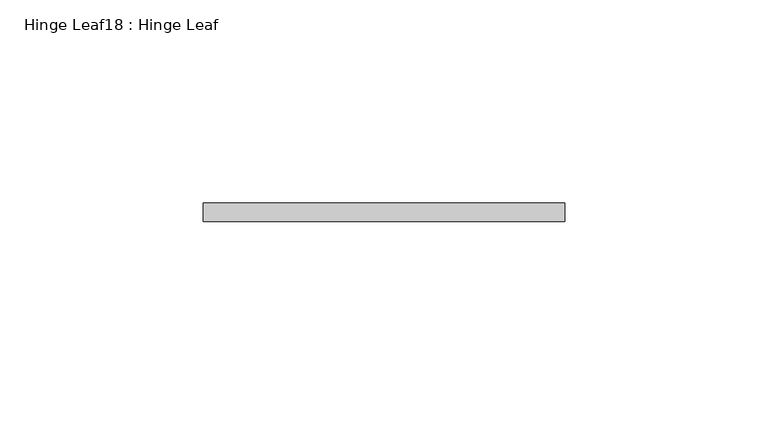
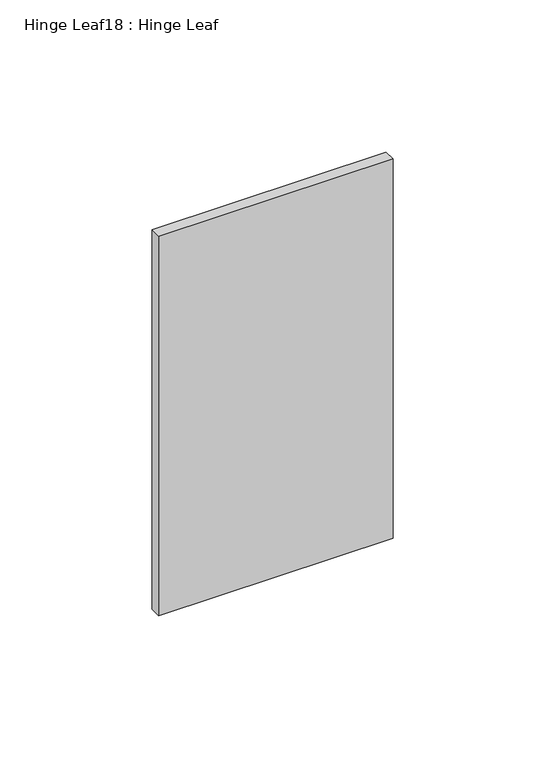
"""IFC4 building model written with IfcOpenShell, lengths in millimetres: proxy geometry, Hinge Leaf18 : Hinge Leaf."""

from ifc_helpers import new_model, si_unit, frame, origin, place, context, project, spatial, polyline, outline, extrude, source, transform, mapped, element, save


def hinge_leaf18_hinge_leaf_9b6187f5(model_context):
    return source(origin(), model_context, "Body", "SweptSolid", [
        extrude(outline(polyline([(587327.7934739, -534104.7943841), (587416.6934739, -534104.7943841), (587416.6934739, -534109.3663841), (587327.7934739, -534109.3663841), (587327.7934739, -534104.7943841)])), frame((0.0, 0.0, 1123.95), z_axis=(0.0, 0.0, 1.0), x_axis=(1.0, 0.0, 0.0)), (0.0, 0.0, 1.0), 152.4),
    ])


if __name__ == "__main__":
    model = new_model("IFC4")
    model_context = context("Model", 3, world=origin())
    ifc_project = project(units=[si_unit("LENGTHUNIT", "METRE", prefix="MILLI")], contexts=[model_context])
    site = spatial("IfcSite", under=ifc_project)
    building = spatial("IfcBuilding", under=site)
    placement = place(None, origin())
    hinge_leaf18_hinge_leaf_shape = hinge_leaf18_hinge_leaf_9b6187f5(model_context)
    element("IfcBuildingElementProxy", 1, Name="Hinge Leaf18 : Hinge Leaf", ObjectType="Hinge Leaf18 : Hinge Leaf", at=placement, inside=building, context=model_context, shape_type="MappedRepresentation", body=[
        mapped(hinge_leaf18_hinge_leaf_shape, transform((0.0, 0.0, 0.0), x_axis=(1.0, 0.0, 0.0), y_axis=(0.0, 1.0, 0.0), z_axis=(0.0, 0.0, 1.0))),
    ])
    save(model, "model.ifc")

# Revit data of these elements
# Element 1 (IfcBuildingElementProxy, "Hinge Leaf18 : Hinge Leaf")
#   Materials on its faces: "6\"X6\" WELD-ON STL BUTT HINGE"
# Materials
#   "6\"X6\" WELD-ON STL BUTT HINGE": class "Metal", colour RGB 189 187 185, transparency 0, Description = "Carbon steel", Cost = 0
